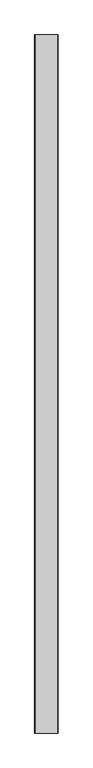
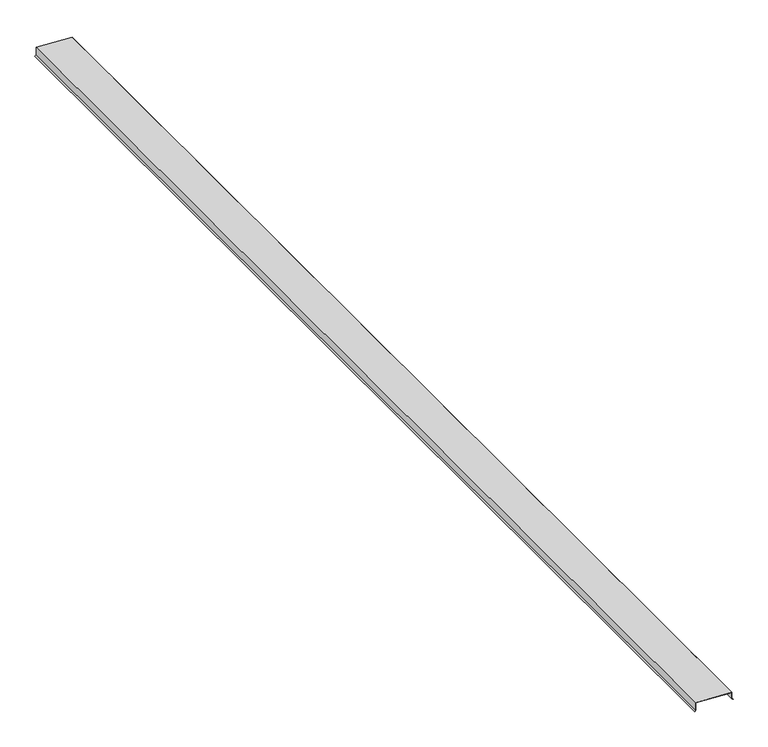
"""IFC4 building model written with IfcOpenShell, lengths in millimetres: proxy geometry, Generic Models 7:Generic Models 1:5:Generic Models 1:5 : Generic Models 7:Generic Models 1:337419:21 : Generic Models 7:Generic Models 1:5:Generic Models 1:5 : Generic Models 7:Generic Models 1:337419:311462."""

import ifcopenshell
import ifcopenshell.guid

model = None  # the IFC model being written
_history = None  # IfcOwnerHistory: only IFC2X3 demands one
_inside = {}  # id of a spatial element -> (the spatial element, [elements in it])
_under = {}  # id of a project, library or spatial element -> (it, [spatial elements below it])
_declared = {}  # id of a project -> (the project, [libraries it declares])
_typed = {}  # id of a type object -> (the type object, [elements of that type])
_made_of = {}  # id of a material, layer set ... -> (it, [elements and type objects made of it])


def new_model(schema):
    """Start an empty IFC model of exactly this schema.

    Asked for "IFC4X3", IfcOpenShell would pick the latest addendum, in which some entities
    have other attributes; the version numbers below select the first issue.
    IFC2X3 requires an IfcOwnerHistory on every rooted entity: one is made here for all.
    """
    global model, _history
    if schema == "IFC4X3":
        model = ifcopenshell.file(schema_version=(4, 3, 0, 0))
    else:
        model = ifcopenshell.file(schema=schema)
    _inside.clear()
    _under.clear()
    _declared.clear()
    _typed.clear()
    _made_of.clear()
    _history = None
    if model.schema == "IFC2X3":
        org = make("IfcOrganization", Name="unknown")
        user = make(
            "IfcPersonAndOrganization",
            ThePerson=make("IfcPerson", FamilyName="unknown"),
            TheOrganization=org,
        )
        app = make(
            "IfcApplication",
            ApplicationDeveloper=org,
            Version="unknown",
            ApplicationFullName="unknown",
            ApplicationIdentifier="unknown",
        )
        _history = make(
            "IfcOwnerHistory",
            OwningUser=user,
            OwningApplication=app,
            ChangeAction="ADDED",
            CreationDate=0,
        )
    return model


def make(cls, **values):
    """One entity of the class cls with the attributes given. An attribute that is None is left unset."""
    return model.create_entity(
        cls, **{name: value for name, value in values.items() if value is not None}
    )


def rooted(cls, **values):
    """An entity with a GlobalId (a new one), such as an element, a storey or a relation."""
    return make(cls, GlobalId=ifcopenshell.guid.new(), OwnerHistory=_history, **values)


def si_unit(unit_type, name, prefix=None):
    """IfcSIUnit, for example si_unit("LENGTHUNIT", "METRE", prefix="MILLI")."""
    return make("IfcSIUnit", UnitType=unit_type, Prefix=prefix, Name=name)


def assignment(units):
    """IfcUnitAssignment: the units of a project."""
    return None if units is None else make("IfcUnitAssignment", Units=units)


def point(xyz):
    """IfcCartesianPoint."""
    return None if xyz is None else make("IfcCartesianPoint", Coordinates=xyz)


def direction(xyz):
    """IfcDirection."""
    return None if xyz is None else make("IfcDirection", DirectionRatios=xyz)


def frame(location, z_axis=None, x_axis=None):
    """IfcAxis2Placement3D, a coordinate frame: its origin and axes. An axis left out is left unset."""
    return make(
        "IfcAxis2Placement3D",
        Location=point(location),
        Axis=direction(z_axis),
        RefDirection=direction(x_axis),
    )


def origin():
    """The frame at (0, 0, 0) with its axes left unset."""
    return frame((0.0, 0.0, 0.0))


def place(relative_to, where):
    """IfcLocalPlacement: puts the frame where relative to a parent placement (None: the world)."""
    return make(
        "IfcLocalPlacement", PlacementRelTo=relative_to, RelativePlacement=where
    )


def context(
    kind, dimensions, precision=None, world=None, true_north=None, identifier=None
):
    """IfcGeometricRepresentationContext, for example the 3D "Model" context."""
    return make(
        "IfcGeometricRepresentationContext",
        ContextIdentifier=identifier,
        ContextType=kind,
        CoordinateSpaceDimension=dimensions,
        Precision=precision,
        WorldCoordinateSystem=world,
        TrueNorth=true_north,
    )


def project(units=None, contexts=None):
    """IfcProject with its units and contexts."""
    return rooted(
        "IfcProject",
        Name="project",
        RepresentationContexts=contexts,
        UnitsInContext=assignment(units),
    )


def spatial(cls, under=None, at=None, **own):
    """A site, building, storey or space (cls), placed at a placement, below another one or the project."""
    s = rooted(cls, ObjectPlacement=at, **own)
    if under is not None:
        _under.setdefault(under.id(), (under, []))[1].append(s)
    return s


def polyline(points):
    """IfcPolyline through the points."""
    return make("IfcPolyline", Points=[point(p) for p in points])


def outline(outer, holes=None, kind="AREA"):
    """IfcArbitraryClosedProfileDef: a profile drawn as a closed curve; with holes, ...WithVoids."""
    if holes is None:
        return make("IfcArbitraryClosedProfileDef", ProfileType=kind, OuterCurve=outer)
    return make(
        "IfcArbitraryProfileDefWithVoids",
        ProfileType=kind,
        OuterCurve=outer,
        InnerCurves=holes,
    )


def extrude(swept, where, along, depth):
    """IfcExtrudedAreaSolid: the profile swept, set in the frame where, extruded along a direction by depth."""
    return make(
        "IfcExtrudedAreaSolid",
        SweptArea=swept,
        Position=where,
        ExtrudedDirection=direction(along),
        Depth=depth,
    )


def shape(context_of_items, identifier, shape_type, items):
    """IfcShapeRepresentation: the items that make up one representation, for example the "Body"."""
    return make(
        "IfcShapeRepresentation",
        ContextOfItems=context_of_items,
        RepresentationIdentifier=identifier,
        RepresentationType=shape_type,
        Items=items,
    )


def source(mapping_origin, context_of_items, identifier, shape_type, items):
    """IfcRepresentationMap: a shape defined once, which mapped items show again and again."""
    return make(
        "IfcRepresentationMap",
        MappingOrigin=mapping_origin,
        MappedRepresentation=shape(context_of_items, identifier, shape_type, items),
    )


def transform(
    local_origin,
    x_axis=None,
    y_axis=None,
    z_axis=None,
    scale=None,
    scale2=None,
    scale3=None,
    uniform=True,
):
    """IfcCartesianTransformationOperator3D, or its non-uniform kind. x_axis, y_axis, z_axis: its Axis1, 2, 3."""
    if uniform:
        return make(
            "IfcCartesianTransformationOperator3D",
            Axis1=direction(x_axis),
            Axis2=direction(y_axis),
            LocalOrigin=point(local_origin),
            Scale=scale,
            Axis3=direction(z_axis),
        )
    return make(
        "IfcCartesianTransformationOperator3DnonUniform",
        Axis1=direction(x_axis),
        Axis2=direction(y_axis),
        LocalOrigin=point(local_origin),
        Scale=scale,
        Axis3=direction(z_axis),
        Scale2=scale2,
        Scale3=scale3,
    )


def mapped(mapping_source, mapping_target):
    """IfcMappedItem: shows the shape of a source again, moved by a transform."""
    return make(
        "IfcMappedItem", MappingSource=mapping_source, MappingTarget=mapping_target
    )


def made_of(thing, what):
    """Note that an element or type object is made of a material, layer set ...; save() writes the relation."""
    if what is not None:
        _made_of.setdefault(what.id(), (what, []))[1].append(thing)
    return thing


def element(
    cls,
    number,
    at=None,
    inside=None,
    cuts=None,
    type_object=None,
    material=None,
    context=None,
    identifier="Body",
    shape_type=None,
    held_by="IfcProductDefinitionShape",
    body=None,
    shapes=None,
    **own,
):
    """One element of the class cls, such as IfcWall. Its Tag is "e" and its number.

    at: its placement. inside: the storey or other place that contains it. cuts: it is an
    opening in that element (IfcRelVoidsElement). A single representation is given by context,
    identifier, shape_type and body (its items); several are given by shapes. held_by: the class
    of the entity that holds the representations. save() writes the other relations.
    """
    e = rooted(cls, Tag="e%d" % number, ObjectPlacement=at, **own)
    if body is not None:
        shapes = [shape(context, identifier, shape_type, body)]
    if shapes is not None:
        e.Representation = make(held_by, Representations=shapes)
    if inside is not None:
        _inside.setdefault(inside.id(), (inside, []))[1].append(e)
    if cuts is not None:
        rooted(
            "IfcRelVoidsElement", RelatingBuildingElement=cuts, RelatedOpeningElement=e
        )
    if type_object is not None:
        _typed.setdefault(type_object.id(), (type_object, []))[1].append(e)
    return made_of(e, material)


def aggregate(whole, parts):
    """IfcRelAggregates: a whole, such as a stair, and the parts it consists of."""
    return rooted("IfcRelAggregates", RelatingObject=whole, RelatedObjects=parts)


def save(model, path):
    """Write the relations noted so far, then the file.

    IfcRelAggregates (storeys below a building ...), IfcRelContainedInSpatialStructure (elements
    in a storey), IfcRelDefinesByType, IfcRelAssociatesMaterial and IfcRelDeclares: one each for
    every whole, place, type object, material and project.
    """
    for whole, parts in _under.values():
        aggregate(whole, parts)
    for where, things in _inside.values():
        rooted(
            "IfcRelContainedInSpatialStructure",
            RelatedElements=things,
            RelatingStructure=where,
        )
    for kind, things in _typed.values():
        rooted("IfcRelDefinesByType", RelatedObjects=things, RelatingType=kind)
    for what, things in _made_of.values():
        rooted("IfcRelAssociatesMaterial", RelatedObjects=things, RelatingMaterial=what)
    for by, libraries in _declared.values():
        rooted("IfcRelDeclares", RelatingContext=by, RelatedDefinitions=libraries)
    model.write(path)


def generic_models_674099d0(model_context):
    return source(origin(), model_context, "Body", "SweptSolid", [
        extrude(outline(polyline([(6099.8348677, 560243.4242241), (6087.1348677, 560230.7242241), (6086.0123357, 560231.8467561), (6099.1773037, 560245.0117241), (6187.0619918, 560245.0117241), (6166.5954438, 560635.5367241), (6099.1773037, 560635.5367241), (6086.0123357, 560648.701692), (6087.1348677, 560649.8242241), (6099.8348677, 560637.1242241), (6168.101925, 560637.1242241), (6188.7348677, 560243.4242241), (6099.8348677, 560243.4242241)])), frame((0.0, -578916.8945489, 0.0), z_axis=(0.0, 1.0, 0.0), x_axis=(0.0, 0.0, 1.0)), (0.0, 0.0, 1.0), 12447.9281647),
    ])


if __name__ == "__main__":
    model = new_model("IFC4")
    model_context = context("Model", 3, world=origin())
    ifc_project = project(units=[si_unit("LENGTHUNIT", "METRE", prefix="MILLI")], contexts=[model_context])
    site = spatial("IfcSite", under=ifc_project)
    building = spatial("IfcBuilding", under=site)
    placement = place(None, origin())
    generic_models_shape = generic_models_674099d0(model_context)
    element("IfcBuildingElementProxy", 1, Name="Generic Models 7:Generic Models 1:5:Generic Models 1:5 : Generic Models 7:Generic Models 1:337419:21 : Generic Models 7:Generic Models 1:5:Generic Models 1:5 : Generic Models 7:Generic Models 1:337419:311462", ObjectType="Generic Models 7:Generic Models 1:5:Generic Models 1:5 : Generic Models 7:Generic Models 1:337419:21 : Generic Models 7:Generic Models 1:5:Generic Models 1:5 : Generic Models 7:Generic Models 1:337419:311462", at=placement, inside=building, context=model_context, shape_type="MappedRepresentation", body=[
        mapped(generic_models_shape, transform((0.0, 0.0, 0.0), x_axis=(1.0, 0.0, 0.0), y_axis=(0.0, 1.0, 0.0), z_axis=(0.0, 0.0, 1.0))),
    ])
    save(model, "model.ifc")

# Revit data of these elements
# Type "Generic Models 7:Generic Models 1:5:Generic Models 1:5 : Generic Models 7:Generic Models 1:337419:21 : Generic Models 7:Generic Models 1:5:Generic Models 1:5 : Generic Models 7:Generic Models 1:337419:311462"
#   NameOverride = "Generic Models 7:Generic Models 1:5:Generic Models 1:5 : Generic Models 7:Generic Models 1:337419:311462"
#   ObjectTypeOverride = "Generic Models 1:5 : Generic Models 7:Generic Models 1:337419"
#   Reference = "Generic Models 1"
#   Tag = "311462"
# Element 1 (IfcBuildingElementProxy, "Generic Models 7:Generic Models 1:5:Generic Models 1:5 : Generic Models 7:Generic Models 1:337419:21 : Generic Models 7:Generic Models 1:5:Generic Models 1:5 : Generic Models 7:Generic Models 1:337419:311462")
#   Materials on its faces: "SHEET METAL COPING (COLOR TO MATCH RESIN PANEL)"
# Materials
#   "SHEET METAL COPING (COLOR TO MATCH RESIN PANEL)": class "Generic", colour RGB 240 240 240, transparency 0, Keynote = "M07711300.01", Cost = 0
